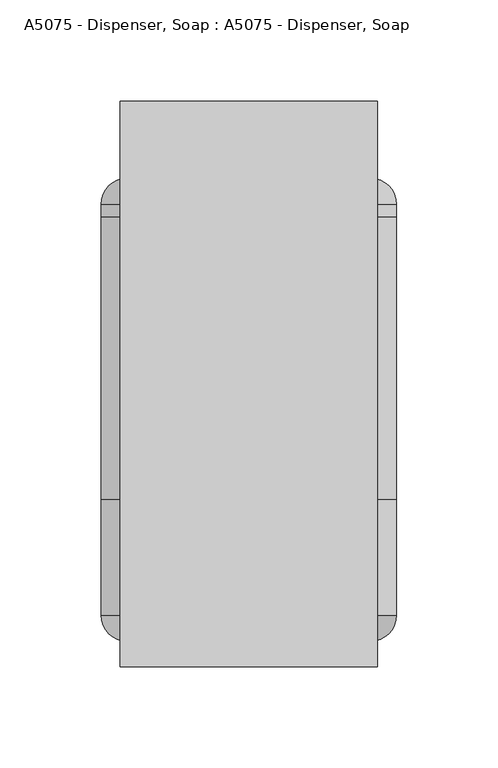
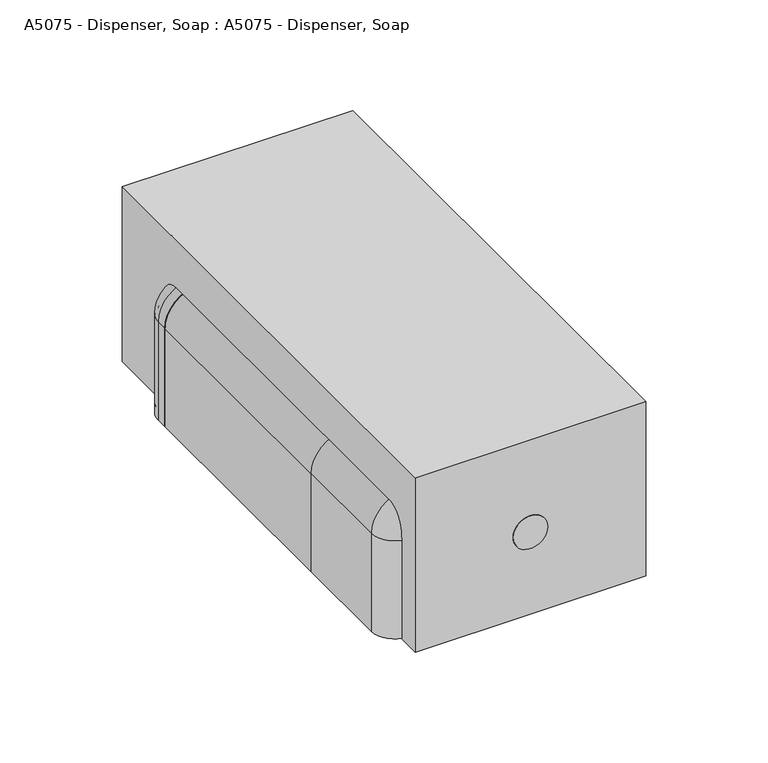
"""IFC4 building model written with IfcOpenShell, lengths in millimetres: proxy geometry, A5075 - Dispenser, Soap : A5075 - Dispenser, Soap."""

import ifcopenshell
import ifcopenshell.guid

model = None  # the IFC model being written
_history = None  # IfcOwnerHistory: only IFC2X3 demands one
_inside = {}  # id of a spatial element -> (the spatial element, [elements in it])
_under = {}  # id of a project, library or spatial element -> (it, [spatial elements below it])
_declared = {}  # id of a project -> (the project, [libraries it declares])
_typed = {}  # id of a type object -> (the type object, [elements of that type])
_made_of = {}  # id of a material, layer set ... -> (it, [elements and type objects made of it])


def new_model(schema):
    """Start an empty IFC model of exactly this schema.

    Asked for "IFC4X3", IfcOpenShell would pick the latest addendum, in which some entities
    have other attributes; the version numbers below select the first issue.
    IFC2X3 requires an IfcOwnerHistory on every rooted entity: one is made here for all.
    """
    global model, _history
    if schema == "IFC4X3":
        model = ifcopenshell.file(schema_version=(4, 3, 0, 0))
    else:
        model = ifcopenshell.file(schema=schema)
    _inside.clear()
    _under.clear()
    _declared.clear()
    _typed.clear()
    _made_of.clear()
    _history = None
    if model.schema == "IFC2X3":
        org = make("IfcOrganization", Name="unknown")
        user = make(
            "IfcPersonAndOrganization",
            ThePerson=make("IfcPerson", FamilyName="unknown"),
            TheOrganization=org,
        )
        app = make(
            "IfcApplication",
            ApplicationDeveloper=org,
            Version="unknown",
            ApplicationFullName="unknown",
            ApplicationIdentifier="unknown",
        )
        _history = make(
            "IfcOwnerHistory",
            OwningUser=user,
            OwningApplication=app,
            ChangeAction="ADDED",
            CreationDate=0,
        )
    return model


def make(cls, **values):
    """One entity of the class cls with the attributes given. An attribute that is None is left unset."""
    return model.create_entity(
        cls, **{name: value for name, value in values.items() if value is not None}
    )


def rooted(cls, **values):
    """An entity with a GlobalId (a new one), such as an element, a storey or a relation."""
    return make(cls, GlobalId=ifcopenshell.guid.new(), OwnerHistory=_history, **values)


def si_unit(unit_type, name, prefix=None):
    """IfcSIUnit, for example si_unit("LENGTHUNIT", "METRE", prefix="MILLI")."""
    return make("IfcSIUnit", UnitType=unit_type, Prefix=prefix, Name=name)


def assignment(units):
    """IfcUnitAssignment: the units of a project."""
    return None if units is None else make("IfcUnitAssignment", Units=units)


def point(xyz):
    """IfcCartesianPoint."""
    return None if xyz is None else make("IfcCartesianPoint", Coordinates=xyz)


def direction(xyz):
    """IfcDirection."""
    return None if xyz is None else make("IfcDirection", DirectionRatios=xyz)


def frame(location, z_axis=None, x_axis=None):
    """IfcAxis2Placement3D, a coordinate frame: its origin and axes. An axis left out is left unset."""
    return make(
        "IfcAxis2Placement3D",
        Location=point(location),
        Axis=direction(z_axis),
        RefDirection=direction(x_axis),
    )


def frame_2d(location, x_axis=None):
    """IfcAxis2Placement2D, a coordinate frame in the plane: its origin and x axis."""
    return make(
        "IfcAxis2Placement2D", Location=point(location), RefDirection=direction(x_axis)
    )


def origin():
    """The frame at (0, 0, 0) with its axes left unset."""
    return frame((0.0, 0.0, 0.0))


def origin_with_axes():
    """The frame at (0, 0, 0) with the z axis (0, 0, 1) and the x axis (1, 0, 0) written out."""
    return frame((0.0, 0.0, 0.0), z_axis=(0.0, 0.0, 1.0), x_axis=(1.0, 0.0, 0.0))


def place(relative_to, where):
    """IfcLocalPlacement: puts the frame where relative to a parent placement (None: the world)."""
    return make(
        "IfcLocalPlacement", PlacementRelTo=relative_to, RelativePlacement=where
    )


def context(
    kind, dimensions, precision=None, world=None, true_north=None, identifier=None
):
    """IfcGeometricRepresentationContext, for example the 3D "Model" context."""
    return make(
        "IfcGeometricRepresentationContext",
        ContextIdentifier=identifier,
        ContextType=kind,
        CoordinateSpaceDimension=dimensions,
        Precision=precision,
        WorldCoordinateSystem=world,
        TrueNorth=true_north,
    )


def project(units=None, contexts=None):
    """IfcProject with its units and contexts."""
    return rooted(
        "IfcProject",
        Name="project",
        RepresentationContexts=contexts,
        UnitsInContext=assignment(units),
    )


def spatial(cls, under=None, at=None, **own):
    """A site, building, storey or space (cls), placed at a placement, below another one or the project."""
    s = rooted(cls, ObjectPlacement=at, **own)
    if under is not None:
        _under.setdefault(under.id(), (under, []))[1].append(s)
    return s


def polyline(points):
    """IfcPolyline through the points."""
    return make("IfcPolyline", Points=[point(p) for p in points])


def circle_curve(where, radius):
    """IfcCircle in the frame where."""
    return make("IfcCircle", Position=where, Radius=radius)


def ellipse_curve(where, semi_axis1, semi_axis2):
    """IfcEllipse in the frame where."""
    return make(
        "IfcEllipse", Position=where, SemiAxis1=semi_axis1, SemiAxis2=semi_axis2
    )


def trimmed(basis, trim1, trim2, sense, master):
    """IfcTrimmedCurve: the piece of a basis curve between two trims."""
    return make(
        "IfcTrimmedCurve",
        BasisCurve=basis,
        Trim1=trim1,
        Trim2=trim2,
        SenseAgreement=sense,
        MasterRepresentation=master,
    )


def segment(curve, same_sense, transition):
    """IfcCompositeCurveSegment."""
    return make(
        "IfcCompositeCurveSegment",
        Transition=transition,
        SameSense=same_sense,
        ParentCurve=curve,
    )


def composite_curve(segments, self_intersect=None):
    """IfcCompositeCurve: segments joined end to end."""
    return make("IfcCompositeCurve", Segments=segments, SelfIntersect=self_intersect)


def outline(outer, holes=None, kind="AREA"):
    """IfcArbitraryClosedProfileDef: a profile drawn as a closed curve; with holes, ...WithVoids."""
    if holes is None:
        return make("IfcArbitraryClosedProfileDef", ProfileType=kind, OuterCurve=outer)
    return make(
        "IfcArbitraryProfileDefWithVoids",
        ProfileType=kind,
        OuterCurve=outer,
        InnerCurves=holes,
    )


def extrude(swept, where, along, depth):
    """IfcExtrudedAreaSolid: the profile swept, set in the frame where, extruded along a direction by depth."""
    return make(
        "IfcExtrudedAreaSolid",
        SweptArea=swept,
        Position=where,
        ExtrudedDirection=direction(along),
        Depth=depth,
    )


def shape(context_of_items, identifier, shape_type, items):
    """IfcShapeRepresentation: the items that make up one representation, for example the "Body"."""
    return make(
        "IfcShapeRepresentation",
        ContextOfItems=context_of_items,
        RepresentationIdentifier=identifier,
        RepresentationType=shape_type,
        Items=items,
    )


def source(mapping_origin, context_of_items, identifier, shape_type, items):
    """IfcRepresentationMap: a shape defined once, which mapped items show again and again."""
    return make(
        "IfcRepresentationMap",
        MappingOrigin=mapping_origin,
        MappedRepresentation=shape(context_of_items, identifier, shape_type, items),
    )


def transform(
    local_origin,
    x_axis=None,
    y_axis=None,
    z_axis=None,
    scale=None,
    scale2=None,
    scale3=None,
    uniform=True,
):
    """IfcCartesianTransformationOperator3D, or its non-uniform kind. x_axis, y_axis, z_axis: its Axis1, 2, 3."""
    if uniform:
        return make(
            "IfcCartesianTransformationOperator3D",
            Axis1=direction(x_axis),
            Axis2=direction(y_axis),
            LocalOrigin=point(local_origin),
            Scale=scale,
            Axis3=direction(z_axis),
        )
    return make(
        "IfcCartesianTransformationOperator3DnonUniform",
        Axis1=direction(x_axis),
        Axis2=direction(y_axis),
        LocalOrigin=point(local_origin),
        Scale=scale,
        Axis3=direction(z_axis),
        Scale2=scale2,
        Scale3=scale3,
    )


def mapped(mapping_source, mapping_target):
    """IfcMappedItem: shows the shape of a source again, moved by a transform."""
    return make(
        "IfcMappedItem", MappingSource=mapping_source, MappingTarget=mapping_target
    )


def made_of(thing, what):
    """Note that an element or type object is made of a material, layer set ...; save() writes the relation."""
    if what is not None:
        _made_of.setdefault(what.id(), (what, []))[1].append(thing)
    return thing


def element(
    cls,
    number,
    at=None,
    inside=None,
    cuts=None,
    type_object=None,
    material=None,
    context=None,
    identifier="Body",
    shape_type=None,
    held_by="IfcProductDefinitionShape",
    body=None,
    shapes=None,
    **own,
):
    """One element of the class cls, such as IfcWall. Its Tag is "e" and its number.

    at: its placement. inside: the storey or other place that contains it. cuts: it is an
    opening in that element (IfcRelVoidsElement). A single representation is given by context,
    identifier, shape_type and body (its items); several are given by shapes. held_by: the class
    of the entity that holds the representations. save() writes the other relations.
    """
    e = rooted(cls, Tag="e%d" % number, ObjectPlacement=at, **own)
    if body is not None:
        shapes = [shape(context, identifier, shape_type, body)]
    if shapes is not None:
        e.Representation = make(held_by, Representations=shapes)
    if inside is not None:
        _inside.setdefault(inside.id(), (inside, []))[1].append(e)
    if cuts is not None:
        rooted(
            "IfcRelVoidsElement", RelatingBuildingElement=cuts, RelatedOpeningElement=e
        )
    if type_object is not None:
        _typed.setdefault(type_object.id(), (type_object, []))[1].append(e)
    return made_of(e, material)


def aggregate(whole, parts):
    """IfcRelAggregates: a whole, such as a stair, and the parts it consists of."""
    return rooted("IfcRelAggregates", RelatingObject=whole, RelatedObjects=parts)


def save(model, path):
    """Write the relations noted so far, then the file.

    IfcRelAggregates (storeys below a building ...), IfcRelContainedInSpatialStructure (elements
    in a storey), IfcRelDefinesByType, IfcRelAssociatesMaterial and IfcRelDeclares: one each for
    every whole, place, type object, material and project.
    """
    for whole, parts in _under.values():
        aggregate(whole, parts)
    for where, things in _inside.values():
        rooted(
            "IfcRelContainedInSpatialStructure",
            RelatedElements=things,
            RelatingStructure=where,
        )
    for kind, things in _typed.values():
        rooted("IfcRelDefinesByType", RelatedObjects=things, RelatingType=kind)
    for what, things in _made_of.values():
        rooted("IfcRelAssociatesMaterial", RelatedObjects=things, RelatingMaterial=what)
    for by, libraries in _declared.values():
        rooted("IfcRelDeclares", RelatingContext=by, RelatedDefinitions=libraries)
    model.write(path)


def plane_surface(at):
    """IfcPlane: the flat surface through the origin of the frame at, square to its z axis."""
    return make("IfcPlane", Position=at)


def cylinder_surface(at, radius):
    """IfcCylindricalSurface: all points at the distance radius from the z axis of the frame at."""
    return make("IfcCylindricalSurface", Position=at, Radius=radius)


def revolved_surface(curve, axis_point, axis_direction):
    """IfcSurfaceOfRevolution: the curve turned about the line through axis_point along axis_direction."""
    return make(
        "IfcSurfaceOfRevolution",
        SweptCurve=make("IfcArbitraryOpenProfileDef", ProfileType="CURVE", Curve=curve),
        AxisPosition=make("IfcAxis1Placement", Location=point(axis_point), Axis=direction(axis_direction)),
    )


def advanced_brep(points, edges, surfaces, faces):
    """IfcAdvancedBrep: a solid bounded by faces that lie on surfaces and meet in shared edges.

    An edge is (start, end): straight between two places in points (the first is 0);
    or (start, end, curve); or (start, end, curve, False) where it runs against its curve.
    A face is (place in surfaces, loops), or (place, loops, False) where it looks against
    its surface's normal. A loop lists edges by number (the first is 1), with a minus sign
    where the edge is run from its end to its start. The first loop is the outer one.
    """
    corners = [point(p) for p in points]
    vertices = [make("IfcVertexPoint", VertexGeometry=c) for c in corners]
    made = []
    for start, end, *more in edges:
        made.append(
            make(
                "IfcEdgeCurve",
                EdgeStart=vertices[start],
                EdgeEnd=vertices[end],
                EdgeGeometry=more[0] if more else make("IfcPolyline", Points=[corners[start], corners[end]]),
                SameSense=more[1] if len(more) > 1 else True,
            )
        )
    hull = []
    for where, loops, *sense in faces:
        bounds = []
        for j, loop in enumerate(loops):
            ring = [make("IfcOrientedEdge", EdgeElement=made[abs(k) - 1], Orientation=k > 0) for k in loop]
            bounds.append(
                make(
                    "IfcFaceOuterBound" if j == 0 else "IfcFaceBound",
                    Bound=make("IfcEdgeLoop", EdgeList=ring),
                    Orientation=True,
                )
            )
        hull.append(make("IfcAdvancedFace", Bounds=bounds, FaceSurface=surfaces[where], SameSense=sense[0] if sense else True))
    return make("IfcAdvancedBrep", Outer=make("IfcClosedShell", CfsFaces=hull))


def a5075_dispenser_soap_a5075_dispenser_soap_c3f38053(model_context):
    return source(origin(), model_context, "Body", "SolidModel", [
        advanced_brep(
        [(-73.025, 25.4, 0.0), (-73.025, 82.55, 0.0), (-71.4375, 82.55, 0.0), (-71.4375, 25.4, 0.0), (-60.325, 14.2875, 0.0), (-60.325, 12.7, 0.0), (-73.025, 25.4, 57.15), (-73.025, 82.55, 57.15), (-53.975, 82.55, 76.2), (53.975, 82.55, 76.2), (73.025, 82.55, 57.15), (73.025, 82.55, 12.7), (71.4375, 82.55, 12.7), (71.4375, 82.55, 57.15), (53.975, 82.55, 74.6125), (-53.975, 82.55, 74.6125), (-71.4375, 82.55, 57.15), (-71.4375, 25.4, 57.15), (-60.325, 14.2875, 57.15), (-60.325, 12.7, 57.15), (-53.975, 25.4, 76.2), (-53.975, 25.4, 74.6125), (-53.975, 14.2875, 63.5), (-53.975, 12.7, 63.5), (53.975, 25.4, 76.2), (53.975, 25.4, 74.6125), (53.975, 14.2875, 63.5), (53.975, 12.7, 63.5), (73.025, 25.4, 57.15), (71.4375, 25.4, 57.15), (60.325, 14.2875, 57.15), (60.325, 12.7, 57.15), (73.025, 25.4, 12.7), (60.325, 12.7, 12.7), (60.325, 14.2875, 12.7), (71.4375, 25.4, 12.7)],
        [
            (0, 1),
            (1, 2),
            (2, 3),
            (3, 4, circle_curve(frame((-60.325, 25.4, 0.0), z_axis=(0.0, 0.0, 1.0), x_axis=(1.0, 0.0, 0.0)), 11.1125)),
            (4, 5),
            (5, 0, circle_curve(frame((-60.325, 25.4, 0.0), z_axis=(0.0, 0.0, -1.0), x_axis=(1.0, 0.0, 0.0)), 12.7)),
            (0, 6),
            (6, 7),
            (7, 1),
            (7, 8, circle_curve(frame((-53.975, 82.55, 57.15), z_axis=(0.0, 1.0, 0.0), x_axis=(-1.0, 0.0, 0.0)), 19.05)),
            (8, 9),
            (9, 10, circle_curve(frame((53.975, 82.55, 57.15), z_axis=(0.0, 1.0, 0.0), x_axis=(0.0, 0.0, 1.0)), 19.05)),
            (10, 11),
            (11, 12),
            (12, 13),
            (13, 14, circle_curve(frame((53.975, 82.55, 57.15), z_axis=(0.0, -1.0, 0.0), x_axis=(0.0, 0.0, 1.0)), 17.4625)),
            (14, 15),
            (15, 16, circle_curve(frame((-53.975, 82.55, 57.15), z_axis=(0.0, -1.0, 0.0), x_axis=(-1.0, 0.0, 0.0)), 17.4625)),
            (16, 2),
            (16, 17),
            (17, 3),
            (17, 18, circle_curve(frame((-60.325, 25.4, 57.15), z_axis=(0.0, 0.0, 1.0), x_axis=(1.0, 0.0, 0.0)), 11.1125)),
            (18, 4),
            (18, 19),
            (19, 5),
            (19, 6, circle_curve(frame((-60.325, 25.4, 57.15), z_axis=(0.0, 0.0, -1.0), x_axis=(1.0, 0.0, 0.0)), 12.7)),
            (6, 20, circle_curve(frame((-53.975, 25.4, 57.15), z_axis=(0.0, 1.0, 0.0), x_axis=(-1.0, 0.0, 0.0)), 19.05)),
            (20, 8),
            (21, 17, circle_curve(frame((-53.975, 25.4, 57.15), z_axis=(0.0, -1.0, 0.0), x_axis=(-1.0, 0.0, 0.0)), 17.4625)),
            (15, 21),
            (22, 18, circle_curve(frame((-53.975, 14.2875, 57.15), z_axis=(0.0, -1.0, 0.0), x_axis=(-1.0, 0.0, 0.0)), 6.35)),
            (21, 22, circle_curve(frame((-53.975, 25.4, 63.5), z_axis=(1.0, 0.0, 0.0), x_axis=(0.0, 0.0, -1.0)), 11.1125)),
            (23, 19, circle_curve(frame((-53.975, 12.7, 57.15), z_axis=(0.0, -1.0, 0.0), x_axis=(-1.0, 0.0, 0.0)), 6.35)),
            (22, 23),
            (23, 20, circle_curve(frame((-53.975, 25.4, 63.5), z_axis=(-1.0, 0.0, 0.0), x_axis=(0.0, 0.0, -1.0)), 12.7)),
            (20, 24),
            (24, 9),
            (14, 25),
            (25, 21),
            (25, 26, circle_curve(frame((53.975, 25.4, 63.5), z_axis=(1.0, 0.0, 0.0), x_axis=(0.0, 0.0, -1.0)), 11.1125)),
            (26, 22),
            (26, 27),
            (27, 23),
            (27, 24, circle_curve(frame((53.975, 25.4, 63.5), z_axis=(-1.0, 0.0, 0.0), x_axis=(0.0, 0.0, -1.0)), 12.7)),
            (24, 28, circle_curve(frame((53.975, 25.4, 57.15), z_axis=(0.0, 1.0, 0.0), x_axis=(0.0, 0.0, 1.0)), 19.05)),
            (28, 10),
            (29, 25, circle_curve(frame((53.975, 25.4, 57.15), z_axis=(0.0, -1.0, 0.0), x_axis=(0.0, 0.0, 1.0)), 17.4625)),
            (13, 29),
            (30, 26, circle_curve(frame((53.975, 14.2875, 57.15), z_axis=(0.0, -1.0, 0.0), x_axis=(0.0, 0.0, 1.0)), 6.35)),
            (29, 30, circle_curve(frame((60.325, 25.4, 57.15), z_axis=(0.0, 0.0, -1.0), x_axis=(-1.0, 0.0, 0.0)), 11.1125)),
            (31, 27, circle_curve(frame((53.975, 12.7, 57.15), z_axis=(0.0, -1.0, 0.0), x_axis=(0.0, 0.0, 1.0)), 6.35)),
            (30, 31),
            (31, 28, circle_curve(frame((60.325, 25.4, 57.15), z_axis=(0.0, 0.0, 1.0), x_axis=(-1.0, 0.0, 0.0)), 12.7)),
            (32, 33, circle_curve(frame((60.325, 25.4, 12.7), z_axis=(0.0, 0.0, -1.0), x_axis=(-1.0, 0.0, 0.0)), 12.7)),
            (33, 34),
            (34, 35, circle_curve(frame((60.325, 25.4, 12.7), z_axis=(0.0, 0.0, 1.0), x_axis=(-1.0, 0.0, 0.0)), 11.1125)),
            (35, 12),
            (11, 32),
            (28, 32),
            (35, 29),
            (34, 30),
            (33, 31),
        ],
        [
            plane_surface(frame((-73.025, 12.7, 0.0), z_axis=(0.0, 0.0, -1.0), x_axis=(0.0, 1.0, 0.0))),
            plane_surface(frame((-73.025, 25.4, 0.0), z_axis=(-1.0, 0.0, 0.0), x_axis=(0.0, 0.0, 1.0))),
            plane_surface(frame((-73.025, 82.55, 0.0), z_axis=(0.0, 1.0, 0.0), x_axis=(0.0, 0.0, 1.0))),
            plane_surface(frame((-71.4375, 82.55, 0.0), z_axis=(1.0, 0.0, 0.0), x_axis=(0.0, 0.0, 1.0))),
            revolved_surface(polyline([(-49.212500000000006, 25.4, 57.15), (-49.212500000000006, 25.4, 0.0)]), (-60.325, 25.4, 0.0), (0.0, 0.0, 1.0)),
            plane_surface(frame((-60.325, 14.2875, 0.0), z_axis=(1.0, 0.0, 0.0), x_axis=(0.0, 0.0, 1.0))),
            cylinder_surface(frame((-60.325, 25.4, 0.0), z_axis=(0.0, 0.0, -1.0), x_axis=(1.0, 0.0, 0.0)), 12.7),
            cylinder_surface(frame((-53.975, 12.7, 57.15), z_axis=(0.0, 1.0, 0.0), x_axis=(-1.0, 0.0, 0.0)), 19.05),
            revolved_surface(polyline([(-71.4375, 82.55, 57.15), (-71.4375, 25.4, 57.15)]), (-53.975, 12.7, 57.15), (0.0, 1.0, 0.0)),
            revolved_surface(trimmed(ellipse_curve(frame((-60.325, 25.4, 57.15), z_axis=(0.0, 0.0, 1.0), x_axis=(1.0, 0.0, 0.0)), 11.1125, 11.1125), [point((-71.4375, 25.4, 57.15))], [point((-60.325, 14.2875, 57.15))], True, "CARTESIAN"), (-53.975, 12.7, 57.15), (0.0, 1.0, 0.0)),
            revolved_surface(polyline([(-60.325, 14.2875, 57.15), (-60.325, 12.7, 57.15)]), (-53.975, 12.7, 57.15), (0.0, 1.0, 0.0)),
            revolved_surface(trimmed(ellipse_curve(frame((-60.325, 25.4, 57.15), z_axis=(0.0, 0.0, -1.0), x_axis=(1.0, 0.0, 0.0)), 12.7, 12.7), [point((-60.325, 12.7, 57.15))], [point((-73.025, 25.4, 57.15))], True, "CARTESIAN"), (-53.975, 12.7, 57.15), (0.0, 1.0, 0.0)),
            plane_surface(frame((-53.975, 25.4, 76.2), z_axis=(0.0, 0.0, 1.0), x_axis=(1.0, 0.0, 0.0))),
            plane_surface(frame((-53.975, 82.55, 74.6125), z_axis=(0.0, 0.0, -1.0), x_axis=(1.0, 0.0, 0.0))),
            revolved_surface(polyline([(53.975, 25.4, 52.3875), (-53.975, 25.4, 52.3875)]), (-53.975, 25.4, 63.5), (1.0, 0.0, 0.0)),
            plane_surface(frame((-53.975, 14.2875, 63.5), z_axis=(0.0, 0.0, -1.0), x_axis=(1.0, 0.0, 0.0))),
            cylinder_surface(frame((-53.975, 25.4, 63.5), z_axis=(-1.0, 0.0, 0.0), x_axis=(0.0, 0.0, -1.0)), 12.7),
            cylinder_surface(frame((53.975, 12.7, 57.15), z_axis=(0.0, 1.0, 0.0), x_axis=(0.0, 0.0, 1.0)), 19.05),
            revolved_surface(polyline([(53.975, 82.55, 74.6125), (53.975, 25.4, 74.6125)]), (53.975, 12.7, 57.15), (0.0, 1.0, 0.0)),
            revolved_surface(trimmed(ellipse_curve(frame((53.975, 25.4, 63.5), z_axis=(1.0, 0.0, 0.0), x_axis=(0.0, 0.0, -1.0)), 11.1125, 11.1125), [point((53.975, 25.4, 74.6125))], [point((53.975, 14.2875, 63.5))], True, "CARTESIAN"), (53.975, 12.7, 57.15), (0.0, 1.0, 0.0)),
            revolved_surface(polyline([(53.975, 14.2875, 63.5), (53.975, 12.7, 63.5)]), (53.975, 12.7, 57.15), (0.0, 1.0, 0.0)),
            revolved_surface(trimmed(ellipse_curve(frame((53.975, 25.4, 63.5), z_axis=(-1.0, 0.0, 0.0), x_axis=(0.0, 0.0, -1.0)), 12.7, 12.7), [point((53.975, 12.7, 63.5))], [point((53.975, 25.4, 76.2))], True, "CARTESIAN"), (53.975, 12.7, 57.15), (0.0, 1.0, 0.0)),
            plane_surface(frame((73.025, 12.7, 12.7), z_axis=(0.0, 0.0, -1.0), x_axis=(0.0, 1.0, 0.0))),
            plane_surface(frame((73.025, 25.4, 57.15), z_axis=(1.0, 0.0, 0.0), x_axis=(0.0, 0.0, -1.0))),
            plane_surface(frame((71.4375, 82.55, 57.15), z_axis=(-1.0, 0.0, 0.0), x_axis=(0.0, 0.0, -1.0))),
            revolved_surface(polyline([(49.212500000000006, 25.4, 12.699999999999996), (49.212500000000006, 25.4, 57.15)]), (60.325, 25.4, 57.15), (0.0, 0.0, -1.0)),
            plane_surface(frame((60.325, 14.2875, 57.15), z_axis=(-1.0, 0.0, 0.0), x_axis=(0.0, 0.0, -1.0))),
            cylinder_surface(frame((60.325, 25.4, 57.15), z_axis=(0.0, 0.0, 1.0), x_axis=(-1.0, 0.0, 0.0)), 12.7),
        ],
        [
            (0, [[1, 2, 3, 4, 5, 6]]),
            (1, [[-1, 7, 8, 9]]),
            (2, [[-2, -9, 10, 11, 12, 13, 14, 15, 16, 17, 18, 19]]),
            (3, [[-3, -19, 20, 21]]),
            (4, [[-4, -21, 22, 23]]),
            (5, [[-5, -23, 24, 25]]),
            (6, [[-6, -25, 26, -7]]),
            (7, [[-10, -8, 27, 28]]),
            (8, [[29, -20, -18, 30]]),
            (9, [[31, -22, -29, 32]]),
            (10, [[33, -24, -31, 34]]),
            (11, [[-27, -26, -33, 35]]),
            (12, [[-28, 36, 37, -11]]),
            (13, [[-30, -17, 38, 39]]),
            (14, [[-32, -39, 40, 41]]),
            (15, [[-34, -41, 42, 43]]),
            (16, [[-35, -43, 44, -36]]),
            (17, [[-12, -37, 45, 46]]),
            (18, [[47, -38, -16, 48]]),
            (19, [[49, -40, -47, 50]]),
            (20, [[51, -42, -49, 52]]),
            (21, [[-45, -44, -51, 53]]),
            (22, [[54, 55, 56, 57, -14, 58]]),
            (23, [[-46, 59, -58, -13]]),
            (24, [[-48, -15, -57, 60]]),
            (25, [[-50, -60, -56, 61]]),
            (26, [[-52, -61, -55, 62]]),
            (27, [[-53, -62, -54, -59]]),
        ],
    ),
        advanced_brep(
        [(-73.025, 228.6, 0.0), (-60.325, 241.3, 0.0), (-60.325, 239.7125, 0.0), (-71.4375, 228.6, 0.0), (-71.4375, 222.25, 0.0), (-73.025, 222.25, 0.0), (-73.025, 228.6, 57.15), (-60.325, 241.3, 57.15), (-60.325, 239.7125, 57.15), (-71.4375, 228.6, 57.15), (-71.4375, 222.25, 57.15), (-53.975, 222.25, 74.6125), (53.975, 222.25, 74.6125), (71.4375, 222.25, 57.15), (71.4375, 222.25, 12.7), (73.025, 222.25, 12.7), (73.025, 222.25, 57.15), (53.975, 222.25, 76.2), (-53.975, 222.25, 76.2), (-73.025, 222.25, 57.15), (-53.975, 241.3, 63.5), (-53.975, 228.6, 76.2), (-53.975, 239.7125, 63.5), (-53.975, 228.6, 74.6125), (53.975, 228.6, 76.2), (53.975, 241.3, 63.5), (53.975, 239.7125, 63.5), (53.975, 228.6, 74.6125), (60.325, 241.3, 57.15), (73.025, 228.6, 57.15), (60.325, 239.7125, 57.15), (71.4375, 228.6, 57.15), (73.025, 228.6, 12.7), (71.4375, 228.6, 12.7), (60.325, 239.7125, 12.7), (60.325, 241.3, 12.7)],
        [
            (0, 1, circle_curve(frame((-60.325, 228.6, 0.0), z_axis=(0.0, 0.0, -1.0), x_axis=(1.0, 0.0, 0.0)), 12.7)),
            (1, 2),
            (2, 3, circle_curve(frame((-60.325, 228.6, 0.0), z_axis=(0.0, 0.0, 1.0), x_axis=(1.0, 0.0, 0.0)), 11.1125)),
            (3, 4),
            (4, 5),
            (5, 0),
            (0, 6),
            (6, 7, circle_curve(frame((-60.325, 228.6, 57.15), z_axis=(0.0, 0.0, -1.0), x_axis=(1.0, 0.0, 0.0)), 12.7)),
            (7, 1),
            (7, 8),
            (8, 2),
            (8, 9, circle_curve(frame((-60.325, 228.6, 57.15), z_axis=(0.0, 0.0, 1.0), x_axis=(1.0, 0.0, 0.0)), 11.1125)),
            (9, 3),
            (9, 10),
            (10, 4),
            (10, 11, circle_curve(frame((-53.975, 222.25, 57.15), z_axis=(0.0, 1.0, 0.0), x_axis=(-1.0, 0.0, 0.0)), 17.4625)),
            (11, 12),
            (12, 13, circle_curve(frame((53.975, 222.25, 57.15), z_axis=(0.0, 1.0, 0.0), x_axis=(0.0, 0.0, 1.0)), 17.4625)),
            (13, 14),
            (14, 15),
            (15, 16),
            (16, 17, circle_curve(frame((53.975, 222.25, 57.15), z_axis=(0.0, -1.0, 0.0), x_axis=(0.0, 0.0, 1.0)), 19.05)),
            (17, 18),
            (18, 19, circle_curve(frame((-53.975, 222.25, 57.15), z_axis=(0.0, -1.0, 0.0), x_axis=(-1.0, 0.0, 0.0)), 19.05)),
            (19, 5),
            (19, 6),
            (20, 7, circle_curve(frame((-53.975, 241.3, 57.15), z_axis=(0.0, -1.0, 0.0), x_axis=(-1.0, 0.0, 0.0)), 6.35)),
            (6, 21, circle_curve(frame((-53.975, 228.6, 57.15), z_axis=(0.0, 1.0, 0.0), x_axis=(-1.0, 0.0, 0.0)), 19.05)),
            (21, 20, circle_curve(frame((-53.975, 228.6, 63.5), z_axis=(-1.0, 0.0, 0.0), x_axis=(0.0, 0.0, -1.0)), 12.7)),
            (22, 8, circle_curve(frame((-53.975, 239.7125, 57.15), z_axis=(0.0, -1.0, 0.0), x_axis=(-1.0, 0.0, 0.0)), 6.35)),
            (20, 22),
            (23, 9, circle_curve(frame((-53.975, 228.6, 57.15), z_axis=(0.0, -1.0, 0.0), x_axis=(-1.0, 0.0, 0.0)), 17.4625)),
            (22, 23, circle_curve(frame((-53.975, 228.6, 63.5), z_axis=(1.0, 0.0, 0.0), x_axis=(0.0, 0.0, -1.0)), 11.1125)),
            (23, 11),
            (18, 21),
            (21, 24),
            (24, 25, circle_curve(frame((53.975, 228.6, 63.5), z_axis=(-1.0, 0.0, 0.0), x_axis=(0.0, 0.0, -1.0)), 12.7)),
            (25, 20),
            (25, 26),
            (26, 22),
            (26, 27, circle_curve(frame((53.975, 228.6, 63.5), z_axis=(1.0, 0.0, 0.0), x_axis=(0.0, 0.0, -1.0)), 11.1125)),
            (27, 23),
            (27, 12),
            (17, 24),
            (28, 25, circle_curve(frame((53.975, 241.3, 57.15), z_axis=(0.0, -1.0, 0.0), x_axis=(0.0, 0.0, 1.0)), 6.35)),
            (24, 29, circle_curve(frame((53.975, 228.6, 57.15), z_axis=(0.0, 1.0, 0.0), x_axis=(0.0, 0.0, 1.0)), 19.05)),
            (29, 28, circle_curve(frame((60.325, 228.6, 57.15), z_axis=(0.0, 0.0, 1.0), x_axis=(-1.0, 0.0, 0.0)), 12.7)),
            (30, 26, circle_curve(frame((53.975, 239.7125, 57.15), z_axis=(0.0, -1.0, 0.0), x_axis=(0.0, 0.0, 1.0)), 6.35)),
            (28, 30),
            (31, 27, circle_curve(frame((53.975, 228.6, 57.15), z_axis=(0.0, -1.0, 0.0), x_axis=(0.0, 0.0, 1.0)), 17.4625)),
            (30, 31, circle_curve(frame((60.325, 228.6, 57.15), z_axis=(0.0, 0.0, -1.0), x_axis=(-1.0, 0.0, 0.0)), 11.1125)),
            (31, 13),
            (16, 29),
            (32, 15),
            (14, 33),
            (33, 34, circle_curve(frame((60.325, 228.6, 12.7), z_axis=(0.0, 0.0, 1.0), x_axis=(-1.0, 0.0, 0.0)), 11.1125)),
            (34, 35),
            (35, 32, circle_curve(frame((60.325, 228.6, 12.7), z_axis=(0.0, 0.0, -1.0), x_axis=(-1.0, 0.0, 0.0)), 12.7)),
            (29, 32),
            (35, 28),
            (34, 30),
            (33, 31),
        ],
        [
            plane_surface(frame((-73.025, 241.3, 0.0), z_axis=(0.0, 0.0, -1.0), x_axis=(0.0, 1.0, 0.0))),
            cylinder_surface(frame((-60.325, 228.6, 0.0), z_axis=(0.0, 0.0, -1.0), x_axis=(1.0, 0.0, 0.0)), 12.7),
            plane_surface(frame((-60.325, 241.3, 0.0), z_axis=(1.0, 0.0, 0.0), x_axis=(0.0, 0.0, 1.0))),
            revolved_surface(polyline([(-49.212500000000006, 228.6, 57.15), (-49.212500000000006, 228.6, 0.0)]), (-60.325, 228.6, 0.0), (0.0, 0.0, 1.0)),
            plane_surface(frame((-71.4375, 228.6, 0.0), z_axis=(1.0, 0.0, 0.0), x_axis=(0.0, 0.0, 1.0))),
            plane_surface(frame((-71.4375, 222.25, 0.0), z_axis=(0.0, -1.0, 0.0), x_axis=(0.0, 0.0, 1.0))),
            plane_surface(frame((-73.025, 222.25, 0.0), z_axis=(-1.0, 0.0, 0.0), x_axis=(0.0, 0.0, 1.0))),
            revolved_surface(trimmed(ellipse_curve(frame((-60.325, 228.6, 57.15), z_axis=(0.0, 0.0, -1.0), x_axis=(1.0, 0.0, 0.0)), 12.7, 12.7), [point((-73.025, 228.6, 57.15))], [point((-60.325, 241.3, 57.15))], True, "CARTESIAN"), (-53.975, 241.3, 57.15), (0.0, 1.0, 0.0)),
            revolved_surface(polyline([(-60.325, 241.3, 57.15), (-60.325, 239.7125, 57.15)]), (-53.975, 241.3, 57.15), (0.0, 1.0, 0.0)),
            revolved_surface(trimmed(ellipse_curve(frame((-60.325, 228.6, 57.15), z_axis=(0.0, 0.0, 1.0), x_axis=(1.0, 0.0, 0.0)), 11.1125, 11.1125), [point((-60.325, 239.7125, 57.15))], [point((-71.4375, 228.6, 57.15))], True, "CARTESIAN"), (-53.975, 241.3, 57.15), (0.0, 1.0, 0.0)),
            revolved_surface(polyline([(-71.4375, 228.6, 57.15), (-71.4375, 222.25, 57.15)]), (-53.975, 241.3, 57.15), (0.0, 1.0, 0.0)),
            cylinder_surface(frame((-53.975, 241.3, 57.15), z_axis=(0.0, 1.0, 0.0), x_axis=(-1.0, 0.0, 0.0)), 19.05),
            cylinder_surface(frame((-53.975, 228.6, 63.5), z_axis=(-1.0, 0.0, 0.0), x_axis=(0.0, 0.0, -1.0)), 12.7),
            plane_surface(frame((-53.975, 241.3, 63.5), z_axis=(0.0, 0.0, -1.0), x_axis=(1.0, 0.0, 0.0))),
            revolved_surface(polyline([(53.975, 228.6, 52.3875), (-53.975, 228.6, 52.3875)]), (-53.975, 228.6, 63.5), (1.0, 0.0, 0.0)),
            plane_surface(frame((-53.975, 228.6, 74.6125), z_axis=(0.0, 0.0, -1.0), x_axis=(1.0, 0.0, 0.0))),
            plane_surface(frame((-53.975, 222.25, 76.2), z_axis=(0.0, 0.0, 1.0), x_axis=(1.0, 0.0, 0.0))),
            revolved_surface(trimmed(ellipse_curve(frame((53.975, 228.6, 63.5), z_axis=(-1.0, 0.0, 0.0), x_axis=(0.0, 0.0, -1.0)), 12.7, 12.7), [point((53.975, 228.6, 76.2))], [point((53.975, 241.3, 63.5))], True, "CARTESIAN"), (53.975, 241.3, 57.15), (0.0, 1.0, 0.0)),
            revolved_surface(polyline([(53.975, 241.3, 63.5), (53.975, 239.7125, 63.5)]), (53.975, 241.3, 57.15), (0.0, 1.0, 0.0)),
            revolved_surface(trimmed(ellipse_curve(frame((53.975, 228.6, 63.5), z_axis=(1.0, 0.0, 0.0), x_axis=(0.0, 0.0, -1.0)), 11.1125, 11.1125), [point((53.975, 239.7125, 63.5))], [point((53.975, 228.6, 74.6125))], True, "CARTESIAN"), (53.975, 241.3, 57.15), (0.0, 1.0, 0.0)),
            revolved_surface(polyline([(53.975, 228.6, 74.6125), (53.975, 222.25, 74.6125)]), (53.975, 241.3, 57.15), (0.0, 1.0, 0.0)),
            cylinder_surface(frame((53.975, 241.3, 57.15), z_axis=(0.0, 1.0, 0.0), x_axis=(0.0, 0.0, 1.0)), 19.05),
            plane_surface(frame((73.025, 241.3, 12.7), z_axis=(0.0, 0.0, -1.0), x_axis=(0.0, 1.0, 0.0))),
            cylinder_surface(frame((60.325, 228.6, 57.15), z_axis=(0.0, 0.0, 1.0), x_axis=(-1.0, 0.0, 0.0)), 12.7),
            plane_surface(frame((60.325, 241.3, 57.15), z_axis=(-1.0, 0.0, 0.0), x_axis=(0.0, 0.0, -1.0))),
            revolved_surface(polyline([(49.212500000000006, 228.6, 12.699999999999996), (49.212500000000006, 228.6, 57.15)]), (60.325, 228.6, 57.15), (0.0, 0.0, -1.0)),
            plane_surface(frame((71.4375, 228.6, 57.15), z_axis=(-1.0, 0.0, 0.0), x_axis=(0.0, 0.0, -1.0))),
            plane_surface(frame((73.025, 222.25, 57.15), z_axis=(1.0, 0.0, 0.0), x_axis=(0.0, 0.0, -1.0))),
        ],
        [
            (0, [[1, 2, 3, 4, 5, 6]]),
            (1, [[-1, 7, 8, 9]]),
            (2, [[-2, -9, 10, 11]]),
            (3, [[-3, -11, 12, 13]]),
            (4, [[-4, -13, 14, 15]]),
            (5, [[-5, -15, 16, 17, 18, 19, 20, 21, 22, 23, 24, 25]]),
            (6, [[-6, -25, 26, -7]]),
            (7, [[27, -8, 28, 29]]),
            (8, [[30, -10, -27, 31]]),
            (9, [[32, -12, -30, 33]]),
            (10, [[-16, -14, -32, 34]]),
            (11, [[-28, -26, -24, 35]]),
            (12, [[-29, 36, 37, 38]]),
            (13, [[-31, -38, 39, 40]]),
            (14, [[-33, -40, 41, 42]]),
            (15, [[-34, -42, 43, -17]]),
            (16, [[-35, -23, 44, -36]]),
            (17, [[45, -37, 46, 47]]),
            (18, [[48, -39, -45, 49]]),
            (19, [[50, -41, -48, 51]]),
            (20, [[-18, -43, -50, 52]]),
            (21, [[-46, -44, -22, 53]]),
            (22, [[54, -20, 55, 56, 57, 58]]),
            (23, [[-47, 59, -58, 60]]),
            (24, [[-49, -60, -57, 61]]),
            (25, [[-51, -61, -56, 62]]),
            (26, [[-52, -62, -55, -19]]),
            (27, [[-53, -21, -54, -59]]),
        ],
    ),
        extrude(outline(composite_curve([segment(polyline([(57.15, -73.025), (0.0, -73.025), (12.7, -71.4375), (57.15, -71.4375)]), True, "CONTINUOUS"), segment(trimmed(circle_curve(frame_2d((57.15, -53.975)), 17.4625), [point((57.15, -71.4375))], [point((74.6125, -53.975))], True, "CARTESIAN"), True, "CONTINUOUS"), segment(polyline([(74.6125, -53.975), (74.6125, 53.975)]), True, "CONTINUOUS"), segment(trimmed(circle_curve(frame_2d((57.15, 53.975)), 17.4625), [point((74.6125, 53.975))], [point((57.15, 71.4375))], True, "CARTESIAN"), True, "CONTINUOUS"), segment(polyline([(57.15, 71.4375), (12.7, 71.4375), (12.7, 73.025), (57.15, 73.025)]), True, "CONTINUOUS"), segment(trimmed(circle_curve(frame_2d((57.15, 53.975)), 19.05), [point((57.15, 73.025))], [point((76.2, 53.975))], False, "CARTESIAN"), True, "CONTINUOUS"), segment(polyline([(76.2, 53.975), (76.2, -53.975)]), True, "CONTINUOUS"), segment(trimmed(circle_curve(frame_2d((57.15, -53.975)), 19.05), [point((76.2, -53.975))], [point((57.15, -73.025))], False, "CARTESIAN"), True, "CONTINUOUS")], self_intersect=False)), frame((0.0, 82.55, 0.0), z_axis=(0.0, 1.0, 0.0), x_axis=(0.0, 0.0, 1.0)), (0.0, 0.0, 1.0), 139.7),
        extrude(outline(composite_curve([segment(polyline([(74.6125, 53.975), (74.6125, -53.975)]), True, "CONTINUOUS"), segment(trimmed(circle_curve(frame_2d((57.15, -53.975)), 17.4625), [point((74.6125, -53.975))], [point((57.15, -71.4375))], False, "CARTESIAN"), True, "CONTINUOUS"), segment(polyline([(57.15, -71.4375), (12.7, -71.4375), (12.7, 71.4375), (57.15, 71.4375)]), True, "CONTINUOUS"), segment(trimmed(circle_curve(frame_2d((57.15, 53.975)), 17.4625), [point((57.15, 71.4375))], [point((74.6125, 53.975))], False, "CARTESIAN"), True, "CONTINUOUS")], self_intersect=False)), frame((0.0, 82.55, 0.0), z_axis=(0.0, 1.0, 0.0), x_axis=(0.0, 0.0, 1.0)), (0.0, 0.0, 1.0), 101.8530988),
        extrude(outline(composite_curve([segment(trimmed(circle_curve(frame_2d((47.625, 0.0)), 9.525), [point((47.625, -9.525))], [point((47.625, 9.525))], False, "CARTESIAN"), True, "CONTINUOUS"), segment(trimmed(circle_curve(frame_2d((47.625, 0.0)), 9.525), [point((47.625, 9.525))], [point((47.625, -9.525))], False, "CARTESIAN"), True, "CONTINUOUS")], self_intersect=False)), frame((0.0, 0.0, 0.0), z_axis=(0.0, 1.0, 0.0), x_axis=(0.0, 0.0, 1.0)), (0.0, 0.0, 1.0), 12.7),
        extrude(outline(composite_curve([segment(polyline([(-9.525, 50.8), (9.525, 50.8)]), True, "CONTINUOUS"), segment(trimmed(circle_curve(frame_2d((9.525, 41.275)), 9.525), [point((9.525, 50.8))], [point((9.525, 31.75))], False, "CARTESIAN"), True, "CONTINUOUS"), segment(polyline([(9.525, 31.75), (-9.525, 31.75)]), True, "CONTINUOUS"), segment(trimmed(circle_curve(frame_2d((-9.525, 41.275)), 9.525), [point((-9.525, 31.75))], [point((-9.525, 50.8))], False, "CARTESIAN"), True, "CONTINUOUS")], self_intersect=False)), frame((0.0, 0.0, 76.2), z_axis=(0.0, 0.0, 1.0), x_axis=(1.0, 0.0, 0.0)), (0.0, 0.0, 1.0), 12.7),
        extrude(outline(composite_curve([segment(polyline([(12.7, -60.325), (12.7, 60.325), (57.15, 60.325)]), True, "CONTINUOUS"), segment(trimmed(circle_curve(frame_2d((57.15, 53.975)), 6.35), [point((57.15, 60.325))], [point((63.5, 53.975))], False, "CARTESIAN"), True, "CONTINUOUS"), segment(polyline([(63.5, 53.975), (63.5, -53.975)]), True, "CONTINUOUS"), segment(trimmed(circle_curve(frame_2d((57.15, -53.975)), 6.35), [point((63.5, -53.975))], [point((57.15, -60.325))], False, "CARTESIAN"), True, "CONTINUOUS"), segment(polyline([(57.15, -60.325), (12.7, -60.325)]), True, "CONTINUOUS")], self_intersect=False)), frame((0.0, 12.7, 0.0), z_axis=(0.0, 1.0, 0.0), x_axis=(0.0, 0.0, 1.0)), (0.0, 0.0, 1.0), 1.5875),
        extrude(outline(composite_curve([segment(polyline([(-60.325, 241.3), (60.325, 241.3)]), True, "CONTINUOUS"), segment(trimmed(circle_curve(frame_2d((60.325, 228.6)), 12.7), [point((60.325, 241.3))], [point((73.025, 228.6))], False, "CARTESIAN"), True, "CONTINUOUS"), segment(polyline([(73.025, 228.6), (73.025, 25.4)]), True, "CONTINUOUS"), segment(trimmed(circle_curve(frame_2d((60.325, 25.4)), 12.7), [point((73.025, 25.4))], [point((60.325, 12.7))], False, "CARTESIAN"), True, "CONTINUOUS"), segment(polyline([(60.325, 12.7), (-60.325, 12.7)]), True, "CONTINUOUS"), segment(trimmed(circle_curve(frame_2d((-60.325, 25.4)), 12.7), [point((-60.325, 12.7))], [point((-73.025, 25.4))], False, "CARTESIAN"), True, "CONTINUOUS"), segment(polyline([(-73.025, 25.4), (-73.025, 228.6)]), True, "CONTINUOUS"), segment(trimmed(circle_curve(frame_2d((-60.325, 228.6)), 12.7), [point((-73.025, 228.6))], [point((-60.325, 241.3))], False, "CARTESIAN"), True, "CONTINUOUS")], self_intersect=False)), origin_with_axes(), (0.0, 0.0, 1.0), 6.35),
        extrude(outline(polyline([(63.5, 279.4), (63.5, 0.0), (-63.5, 0.0), (-63.5, 279.4), (63.5, 279.4)])), origin_with_axes(), (0.0, 0.0, 1.0), 101.6),
        extrude(outline(composite_curve([segment(polyline([(0.0, -60.325), (0.0, 60.325), (44.45, 60.325)]), True, "CONTINUOUS"), segment(trimmed(circle_curve(frame_2d((44.45, 53.975)), 6.35), [point((44.45, 60.325))], [point((50.8, 53.975))], False, "CARTESIAN"), True, "CONTINUOUS"), segment(polyline([(50.8, 53.975), (50.8, -53.975)]), True, "CONTINUOUS"), segment(trimmed(circle_curve(frame_2d((44.45, -53.975)), 6.35), [point((50.8, -53.975))], [point((44.45, -60.325))], False, "CARTESIAN"), True, "CONTINUOUS"), segment(polyline([(44.45, -60.325), (0.0, -60.325)]), True, "CONTINUOUS")], self_intersect=False)), frame((0.0, 239.7125, 0.0), z_axis=(0.0, 1.0, 0.0), x_axis=(0.0, 0.0, 1.0)), (0.0, 0.0, 1.0), 1.5875),
    ])


if __name__ == "__main__":
    model = new_model("IFC4")
    model_context = context("Model", 3, world=origin())
    ifc_project = project(units=[si_unit("LENGTHUNIT", "METRE", prefix="MILLI")], contexts=[model_context])
    site = spatial("IfcSite", under=ifc_project)
    building = spatial("IfcBuilding", under=site)
    placement = place(None, origin())
    a5075_dispenser_soap_a5075_dispenser_soap_shape = a5075_dispenser_soap_a5075_dispenser_soap_c3f38053(model_context)
    element("IfcBuildingElementProxy", 1, Name="A5075 - Dispenser, Soap : A5075 - Dispenser, Soap", ObjectType="A5075 - Dispenser, Soap : A5075 - Dispenser, Soap", at=placement, inside=building, context=model_context, shape_type="MappedRepresentation", body=[
        mapped(a5075_dispenser_soap_a5075_dispenser_soap_shape, transform((0.0, 0.0, 0.0), x_axis=(1.0, 0.0, 0.0), y_axis=(0.0, 1.0, 0.0), z_axis=(0.0, 0.0, 1.0))),
    ])
    save(model, "model.ifc")

# Revit data of these elements
# Type "A5075 - Dispenser, Soap : A5075 - Dispenser, Soap"
#   Watts2 = "0"
#   Watts1 = "0"
#   Unit_Issue = "EA"
#   UTIL_6_Misc = "-"
#   UTIL_5_NonMedGas = "-"
#   UTIL_4_MiscGas = "-"
#   UTIL_3_MedGas = "-"
#   UTIL_2_Elec = "-"
#   UTIL_1_WaterDrain = "-"
#   Nomenclature = "Dispenser, Soap, Disposable"
#   NSN = "4510"
#   Location [instance default] = ""
#   JSN = "A5075"
#   Fund_Source_VA = "-"
#   Fund_Source_Navy = "-"
#   Fund_Source_Army = "-"
#   Fund_Source_AF = "-"
#   ELEC_Volts2 = "0"
#   ELEC_Volts1 = "0"
#   ELEC_Phase2 = "0"
#   ELEC_Phase1 = "0"
#   ELEC_HertzSwitch = "0"
#   ELEC_HertzDependent = "0"
#   ELEC_Hertz = "0"
#   ELEC_Amps2 = "0"
#   ELEC_Amps1 = "0"
#   DetailDescription = "Disposable soap dispenser. One-handed dispensing operation. Designed to accommodate disposable soap cartridge and valve."
#   CAT_VA = "C"
#   CAT_Navy = "C"
#   CAT_IHS = "-"
#   CAT_Army = "C"
#   CAT_AF = "C"
#   BTUperhour = "0"
#   Weight_IP = 3
#   Default Elevation = 4' - 0"
#   DIM_Width_IP = 0' - 5"
#   DIM_Height_IP = 0' - 11"
#   DIM_Depth_IP = 0' - 4"
#   Assembly Code = ""
# Element 1 (IfcBuildingElementProxy, "A5075 - Dispenser, Soap : A5075 - Dispenser, Soap")
#   Materials on its faces: "White Paint", "Glass", "EquipSpace"
# Materials
#   "White Paint": class "Unassigned", colour RGB 249 249 249, transparency 0
#   "Glass": class "Glass", colour RGB 0 128 192, transparency 0.75
#   "EquipSpace": class "Unassigned", colour RGB 221 217 195, transparency 0.5
